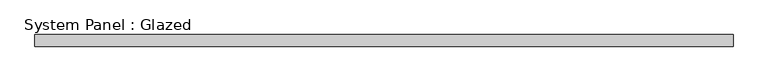
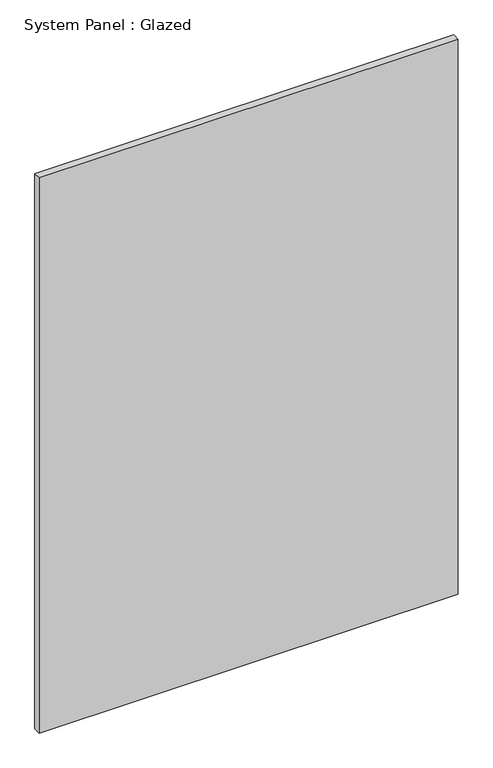
"""IFC4 building model written with IfcOpenShell, lengths in millimetres: plate geometry, System Panel : Glazed."""

import ifcopenshell
import ifcopenshell.guid

model = None  # the IFC model being written
_history = None  # IfcOwnerHistory: only IFC2X3 demands one
_inside = {}  # id of a spatial element -> (the spatial element, [elements in it])
_under = {}  # id of a project, library or spatial element -> (it, [spatial elements below it])
_declared = {}  # id of a project -> (the project, [libraries it declares])
_typed = {}  # id of a type object -> (the type object, [elements of that type])
_made_of = {}  # id of a material, layer set ... -> (it, [elements and type objects made of it])


def new_model(schema):
    """Start an empty IFC model of exactly this schema.

    Asked for "IFC4X3", IfcOpenShell would pick the latest addendum, in which some entities
    have other attributes; the version numbers below select the first issue.
    IFC2X3 requires an IfcOwnerHistory on every rooted entity: one is made here for all.
    """
    global model, _history
    if schema == "IFC4X3":
        model = ifcopenshell.file(schema_version=(4, 3, 0, 0))
    else:
        model = ifcopenshell.file(schema=schema)
    _inside.clear()
    _under.clear()
    _declared.clear()
    _typed.clear()
    _made_of.clear()
    _history = None
    if model.schema == "IFC2X3":
        org = make("IfcOrganization", Name="unknown")
        user = make(
            "IfcPersonAndOrganization",
            ThePerson=make("IfcPerson", FamilyName="unknown"),
            TheOrganization=org,
        )
        app = make(
            "IfcApplication",
            ApplicationDeveloper=org,
            Version="unknown",
            ApplicationFullName="unknown",
            ApplicationIdentifier="unknown",
        )
        _history = make(
            "IfcOwnerHistory",
            OwningUser=user,
            OwningApplication=app,
            ChangeAction="ADDED",
            CreationDate=0,
        )
    return model


def make(cls, **values):
    """One entity of the class cls with the attributes given. An attribute that is None is left unset."""
    return model.create_entity(
        cls, **{name: value for name, value in values.items() if value is not None}
    )


def rooted(cls, **values):
    """An entity with a GlobalId (a new one), such as an element, a storey or a relation."""
    return make(cls, GlobalId=ifcopenshell.guid.new(), OwnerHistory=_history, **values)


def si_unit(unit_type, name, prefix=None):
    """IfcSIUnit, for example si_unit("LENGTHUNIT", "METRE", prefix="MILLI")."""
    return make("IfcSIUnit", UnitType=unit_type, Prefix=prefix, Name=name)


def assignment(units):
    """IfcUnitAssignment: the units of a project."""
    return None if units is None else make("IfcUnitAssignment", Units=units)


def point(xyz):
    """IfcCartesianPoint."""
    return None if xyz is None else make("IfcCartesianPoint", Coordinates=xyz)


def direction(xyz):
    """IfcDirection."""
    return None if xyz is None else make("IfcDirection", DirectionRatios=xyz)


def frame(location, z_axis=None, x_axis=None):
    """IfcAxis2Placement3D, a coordinate frame: its origin and axes. An axis left out is left unset."""
    return make(
        "IfcAxis2Placement3D",
        Location=point(location),
        Axis=direction(z_axis),
        RefDirection=direction(x_axis),
    )


def origin():
    """The frame at (0, 0, 0) with its axes left unset."""
    return frame((0.0, 0.0, 0.0))


def origin_with_axes():
    """The frame at (0, 0, 0) with the z axis (0, 0, 1) and the x axis (1, 0, 0) written out."""
    return frame((0.0, 0.0, 0.0), z_axis=(0.0, 0.0, 1.0), x_axis=(1.0, 0.0, 0.0))


def place(relative_to, where):
    """IfcLocalPlacement: puts the frame where relative to a parent placement (None: the world)."""
    return make(
        "IfcLocalPlacement", PlacementRelTo=relative_to, RelativePlacement=where
    )


def context(
    kind, dimensions, precision=None, world=None, true_north=None, identifier=None
):
    """IfcGeometricRepresentationContext, for example the 3D "Model" context."""
    return make(
        "IfcGeometricRepresentationContext",
        ContextIdentifier=identifier,
        ContextType=kind,
        CoordinateSpaceDimension=dimensions,
        Precision=precision,
        WorldCoordinateSystem=world,
        TrueNorth=true_north,
    )


def project(units=None, contexts=None):
    """IfcProject with its units and contexts."""
    return rooted(
        "IfcProject",
        Name="project",
        RepresentationContexts=contexts,
        UnitsInContext=assignment(units),
    )


def spatial(cls, under=None, at=None, **own):
    """A site, building, storey or space (cls), placed at a placement, below another one or the project."""
    s = rooted(cls, ObjectPlacement=at, **own)
    if under is not None:
        _under.setdefault(under.id(), (under, []))[1].append(s)
    return s


def polyline(points):
    """IfcPolyline through the points."""
    return make("IfcPolyline", Points=[point(p) for p in points])


def outline(outer, holes=None, kind="AREA"):
    """IfcArbitraryClosedProfileDef: a profile drawn as a closed curve; with holes, ...WithVoids."""
    if holes is None:
        return make("IfcArbitraryClosedProfileDef", ProfileType=kind, OuterCurve=outer)
    return make(
        "IfcArbitraryProfileDefWithVoids",
        ProfileType=kind,
        OuterCurve=outer,
        InnerCurves=holes,
    )


def extrude(swept, where, along, depth):
    """IfcExtrudedAreaSolid: the profile swept, set in the frame where, extruded along a direction by depth."""
    return make(
        "IfcExtrudedAreaSolid",
        SweptArea=swept,
        Position=where,
        ExtrudedDirection=direction(along),
        Depth=depth,
    )


def shape(context_of_items, identifier, shape_type, items):
    """IfcShapeRepresentation: the items that make up one representation, for example the "Body"."""
    return make(
        "IfcShapeRepresentation",
        ContextOfItems=context_of_items,
        RepresentationIdentifier=identifier,
        RepresentationType=shape_type,
        Items=items,
    )


def source(mapping_origin, context_of_items, identifier, shape_type, items):
    """IfcRepresentationMap: a shape defined once, which mapped items show again and again."""
    return make(
        "IfcRepresentationMap",
        MappingOrigin=mapping_origin,
        MappedRepresentation=shape(context_of_items, identifier, shape_type, items),
    )


def transform(
    local_origin,
    x_axis=None,
    y_axis=None,
    z_axis=None,
    scale=None,
    scale2=None,
    scale3=None,
    uniform=True,
):
    """IfcCartesianTransformationOperator3D, or its non-uniform kind. x_axis, y_axis, z_axis: its Axis1, 2, 3."""
    if uniform:
        return make(
            "IfcCartesianTransformationOperator3D",
            Axis1=direction(x_axis),
            Axis2=direction(y_axis),
            LocalOrigin=point(local_origin),
            Scale=scale,
            Axis3=direction(z_axis),
        )
    return make(
        "IfcCartesianTransformationOperator3DnonUniform",
        Axis1=direction(x_axis),
        Axis2=direction(y_axis),
        LocalOrigin=point(local_origin),
        Scale=scale,
        Axis3=direction(z_axis),
        Scale2=scale2,
        Scale3=scale3,
    )


def mapped(mapping_source, mapping_target):
    """IfcMappedItem: shows the shape of a source again, moved by a transform."""
    return make(
        "IfcMappedItem", MappingSource=mapping_source, MappingTarget=mapping_target
    )


def made_of(thing, what):
    """Note that an element or type object is made of a material, layer set ...; save() writes the relation."""
    if what is not None:
        _made_of.setdefault(what.id(), (what, []))[1].append(thing)
    return thing


def element(
    cls,
    number,
    at=None,
    inside=None,
    cuts=None,
    type_object=None,
    material=None,
    context=None,
    identifier="Body",
    shape_type=None,
    held_by="IfcProductDefinitionShape",
    body=None,
    shapes=None,
    **own,
):
    """One element of the class cls, such as IfcWall. Its Tag is "e" and its number.

    at: its placement. inside: the storey or other place that contains it. cuts: it is an
    opening in that element (IfcRelVoidsElement). A single representation is given by context,
    identifier, shape_type and body (its items); several are given by shapes. held_by: the class
    of the entity that holds the representations. save() writes the other relations.
    """
    e = rooted(cls, Tag="e%d" % number, ObjectPlacement=at, **own)
    if body is not None:
        shapes = [shape(context, identifier, shape_type, body)]
    if shapes is not None:
        e.Representation = make(held_by, Representations=shapes)
    if inside is not None:
        _inside.setdefault(inside.id(), (inside, []))[1].append(e)
    if cuts is not None:
        rooted(
            "IfcRelVoidsElement", RelatingBuildingElement=cuts, RelatedOpeningElement=e
        )
    if type_object is not None:
        _typed.setdefault(type_object.id(), (type_object, []))[1].append(e)
    return made_of(e, material)


def aggregate(whole, parts):
    """IfcRelAggregates: a whole, such as a stair, and the parts it consists of."""
    return rooted("IfcRelAggregates", RelatingObject=whole, RelatedObjects=parts)


def save(model, path):
    """Write the relations noted so far, then the file.

    IfcRelAggregates (storeys below a building ...), IfcRelContainedInSpatialStructure (elements
    in a storey), IfcRelDefinesByType, IfcRelAssociatesMaterial and IfcRelDeclares: one each for
    every whole, place, type object, material and project.
    """
    for whole, parts in _under.values():
        aggregate(whole, parts)
    for where, things in _inside.values():
        rooted(
            "IfcRelContainedInSpatialStructure",
            RelatedElements=things,
            RelatingStructure=where,
        )
    for kind, things in _typed.values():
        rooted("IfcRelDefinesByType", RelatedObjects=things, RelatingType=kind)
    for what, things in _made_of.values():
        rooted("IfcRelAssociatesMaterial", RelatedObjects=things, RelatingMaterial=what)
    for by, libraries in _declared.values():
        rooted("IfcRelDeclares", RelatingContext=by, RelatedDefinitions=libraries)
    model.write(path)


def system_panel_glazed_baa26042(model_context):
    return source(origin(), model_context, "Body", "SweptSolid", [
        extrude(outline(polyline([(724.9999999, 24.5), (-724.9999999, 24.5), (-724.9999999, 49.5), (724.9999999, 49.5), (724.9999999, 24.5)])), origin_with_axes(), (0.0, 0.0, 1.0), 2030.4462072),
    ])


if __name__ == "__main__":
    model = new_model("IFC4")
    model_context = context("Model", 3, world=origin())
    ifc_project = project(units=[si_unit("LENGTHUNIT", "METRE", prefix="MILLI")], contexts=[model_context])
    site = spatial("IfcSite", under=ifc_project)
    building = spatial("IfcBuilding", under=site)
    placement = place(None, origin())
    system_panel_glazed_shape = system_panel_glazed_baa26042(model_context)
    element("IfcPlate", 1, ObjectType="System Panel : Glazed", at=placement, inside=building, context=model_context, shape_type="MappedRepresentation", body=[
        mapped(system_panel_glazed_shape, transform((0.0, 0.0, 0.0), x_axis=(1.0, 0.0, 0.0), y_axis=(0.0, 1.0, 0.0), z_axis=(0.0, 0.0, 1.0))),
    ])
    save(model, "model.ifc")

# Revit data of these elements
# Type "System Panel : Glazed"
#   Construction Type Id = "GSP4R"
#   Analytic Construction = "1/8 in Pilkington single glazing"
#   Visual Light Transmittance = 0.9
#   Solar Heat Gain Coefficient = 0.86
#   Heat Transfer Coefficient (U) = 6.7069 W/(m²·K)
#   Define Thermal Properties by = 1
# Element 1 (IfcPlate, "System Panel : Glazed")
#   Materials on its faces: "Glass"
# Materials
#   "Glass": class "Glass", colour RGB 0 128 192, transparency 0.9, Description = "Soda Lime Glass", Cost = 0
